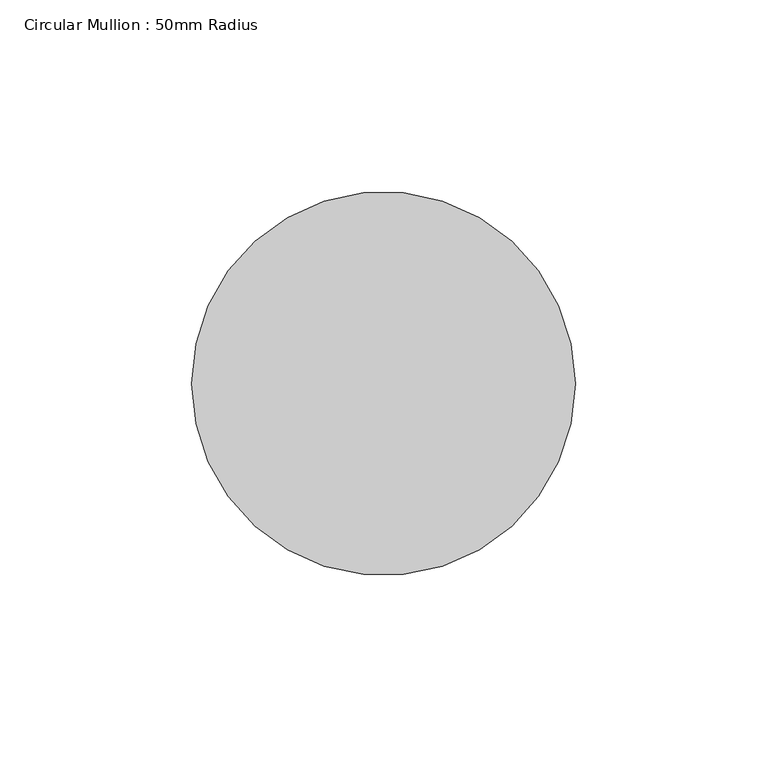
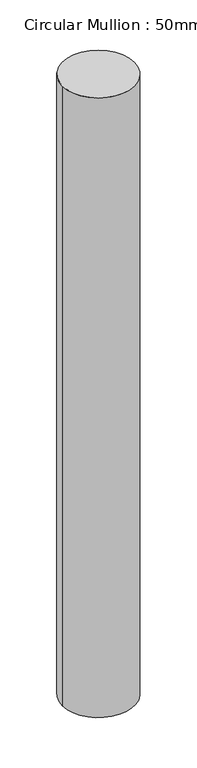
"""IFC4 building model written with IfcOpenShell, lengths in millimetres: member geometry, Circular Mullion : 50mm Radius."""

from ifc_helpers import new_model, si_unit, point, frame, origin, origin_2d, place, context, project, spatial, circle_curve, trimmed, segment, composite_curve, outline, extrude, source, transform, mapped, element, save


def circular_mullion_50mm_radius_ddca1b36(model_context):
    return source(origin(), model_context, "Body", "SweptSolid", [
        extrude(outline(composite_curve([segment(trimmed(circle_curve(origin_2d(), 50.0), [point((50.0, 0.0))], [point((-50.0, 0.0))], False, "CARTESIAN"), True, "CONTINUOUS"), segment(trimmed(circle_curve(origin_2d(), 50.0), [point((-50.0, 0.0))], [point((50.0, 0.0))], False, "CARTESIAN"), True, "CONTINUOUS")], self_intersect=False)), frame((0.0, 0.0, -909.7614818), z_axis=(0.0, 0.0, 1.0), x_axis=(1.0, 0.0, 0.0)), (0.0, 0.0, 1.0), 909.7614818),
    ])


if __name__ == "__main__":
    model = new_model("IFC4")
    model_context = context("Model", 3, world=origin())
    ifc_project = project(units=[si_unit("LENGTHUNIT", "METRE", prefix="MILLI")], contexts=[model_context])
    site = spatial("IfcSite", under=ifc_project)
    building = spatial("IfcBuilding", under=site)
    placement = place(None, origin())
    circular_mullion_50mm_radius_shape = circular_mullion_50mm_radius_ddca1b36(model_context)
    element("IfcMember", 1, ObjectType="Circular Mullion : 50mm Radius", at=placement, inside=building, context=model_context, shape_type="MappedRepresentation", body=[
        mapped(circular_mullion_50mm_radius_shape, transform((0.0, 0.0, 0.0), x_axis=(1.0, 0.0, 0.0), y_axis=(0.0, 1.0, 0.0), z_axis=(0.0, 0.0, 1.0))),
    ])
    save(model, "model.ifc")

# Revit data of these elements
# Type "Circular Mullion : 50mm Radius"
#   built-in parameter 1007350 = 0.164042 (stored number, unit not read)
# Element 1 (IfcMember, "Circular Mullion : 50mm Radius")
#   Materials on its faces: "Aluminium"
# Materials
#   "Aluminium": class "Metal", colour RGB 247 247 247, transparency 0, Description = "Aluminium 6061", Cost = 0
